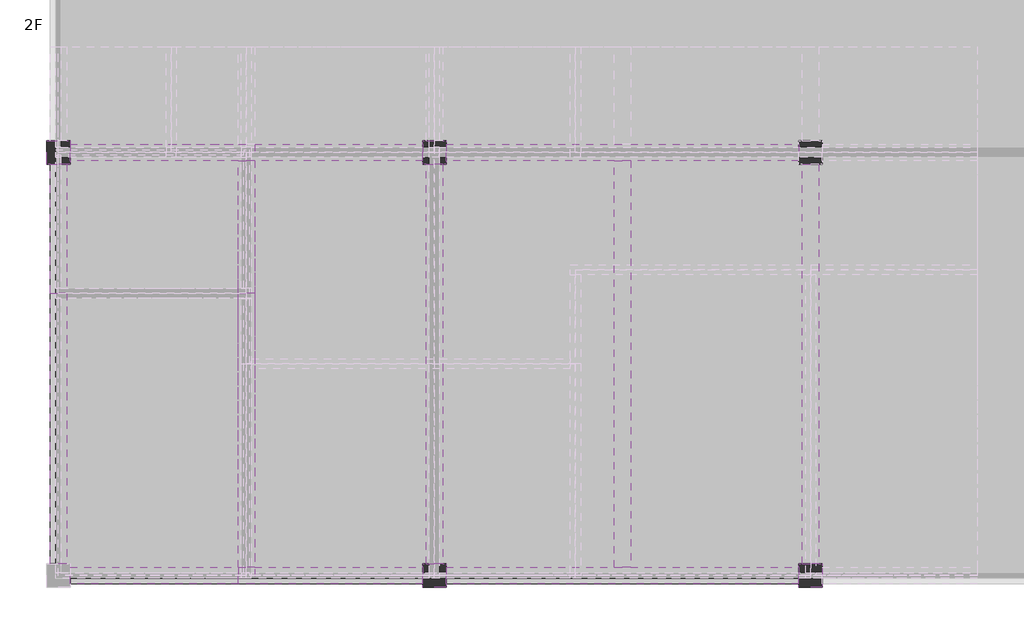
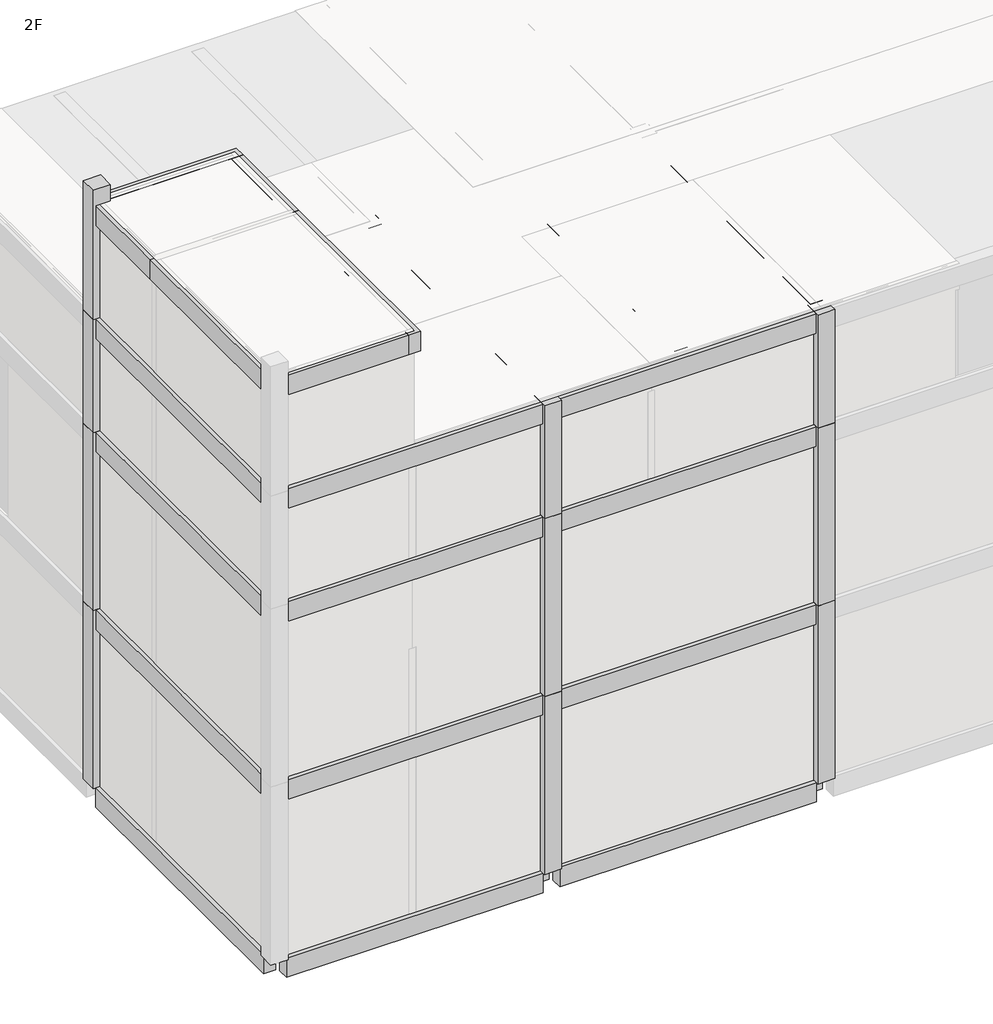
# One storey, part 4 of 7: 42 beams, 14 columns.
"""IFC4 building model written with IfcOpenShell, lengths in millimetres."""

from ifc_helpers import new_model, si_unit, frame, origin, place, context, project, spatial, polyline, outline, extrude, faceted_brep, element, save

model = new_model("IFC4")

# Units and contexts
model_context = context("Model", 3, world=origin())
ifc_project = project(units=[si_unit("LENGTHUNIT", "METRE", prefix="MILLI")], contexts=[model_context])

# Site, building, storey
site = spatial("IfcSite", under=ifc_project)
building = spatial("IfcBuilding", under=site)
storey = spatial("IfcBuildingStorey", under=building, Name="2F", Elevation=3500.0)

# Beams
placement = place(None, origin())
element("IfcBeam", 1, ObjectType="Concrete-Rectangular-Beam : BM111_400x500_RG1", at=placement, inside=storey, context=model_context, shape_type="Brep", body=[
    faceted_brep([(49634.6521483, 169923.8614395, 21500.0), (49284.6521483, 169923.8614395, 21500.0), (49284.6521483, 164098.8614395, 21500.0), (49284.6521483, 163748.8614395, 21500.0), (49634.6521483, 163748.8614395, 21500.0), (49634.6521483, 169923.8614395, 20900.0), (49634.6521483, 163748.8614395, 20900.0), (49284.6521483, 169923.8614395, 20900.0), (49284.6521483, 163748.8614395, 20900.0), (49284.6521483, 164098.8614395, 20900.0)], [[[0, 1, 2, 3, 4]], [[5, 0, 4, 6]], [[7, 5, 6, 8, 9]], [[1, 7, 9, 8, 3, 2]], [[4, 3, 8, 6]], [[1, 0, 5, 7]]]),
])
element("IfcBeam", 2, ObjectType="Concrete-Rectangular-Beam : BM111_400x500_RG1", at=placement, inside=storey, context=model_context, shape_type="SweptSolid", body=[
    extrude(outline(polyline([(49284.6521483, 164098.8614395), (49284.6521483, 163748.8614395), (45709.6521483, 163748.8614395), (45709.6521483, 164098.8614395), (49284.6521483, 164098.8614395)])), frame((0.0, 0.0, 20900.0), z_axis=(0.0, 0.0, 1.0), x_axis=(1.0, 0.0, 0.0)), (0.0, 0.0, 1.0), 600.0),
])
element("IfcBeam", 3, ObjectType="Concrete-Rectangular-Beam : BM111_400x500_RG1", at=placement, inside=storey, context=model_context, shape_type="SweptSolid", body=[
    extrude(outline(polyline([(45284.6521483, 169923.8614395), (45634.6521483, 169923.8614395), (45634.6521483, 164173.8614395), (45284.6521483, 164173.8614395), (45284.6521483, 169923.8614395)])), frame((0.0, 0.0, 20900.0), z_axis=(0.0, 0.0, 1.0), x_axis=(1.0, 0.0, 0.0)), (0.0, 0.0, 1.0), 600.0),
])
element("IfcBeam", 4, ObjectType="Concrete-Rectangular-Beam : BM111_400x500_RG1", at=placement, inside=storey, context=model_context, shape_type="Brep", body=[
    faceted_brep([(49634.6521483, 172748.8614395, 21500.0), (49634.6521483, 173098.8614395, 21500.0), (45709.6521483, 173098.8614395, 21500.0), (45709.6521483, 172748.8614395, 21500.0), (49284.6521483, 172748.8614395, 21500.0), (49634.6521483, 173098.8614395, 20900.0), (45709.6521483, 173098.8614395, 20900.0), (49634.6521483, 172748.8614395, 20900.0), (49284.6521483, 172748.8614395, 20900.0), (45709.6521483, 172748.8614395, 20900.0)], [[[0, 1, 2, 3, 4]], [[1, 5, 6, 2]], [[5, 7, 8, 9, 6]], [[7, 0, 4, 3, 9, 8]], [[3, 2, 6, 9]], [[1, 0, 7, 5]]]),
])
element("IfcBeam", 5, ObjectType="Concrete-Rectangular-Beam : BM111_400x500_RG1", at=placement, inside=storey, context=model_context, shape_type="SweptSolid", body=[
    extrude(outline(polyline([(49634.6521483, 169923.8614395), (49284.6521483, 169923.8614395), (49284.6521483, 172748.8614395), (49634.6521483, 172748.8614395), (49634.6521483, 169923.8614395)])), frame((0.0, 0.0, 20900.0), z_axis=(0.0, 0.0, 1.0), x_axis=(1.0, 0.0, 0.0)), (0.0, 0.0, 1.0), 600.0),
])
element("IfcBeam", 6, ObjectType="Concrete-Rectangular-Beam : BM111_400x500_RG1", at=placement, inside=storey, context=model_context, shape_type="SweptSolid", body=[
    extrude(outline(polyline([(45634.6521483, 169923.8614395), (45284.6521483, 169923.8614395), (45284.6521483, 172673.8614395), (45634.6521483, 172673.8614395), (45634.6521483, 169923.8614395)])), frame((0.0, 0.0, 20900.0), z_axis=(0.0, 0.0, 1.0), x_axis=(1.0, 0.0, 0.0)), (0.0, 0.0, 1.0), 600.0),
])
element("IfcBeam", 7, ObjectType="Concrete-Rectangular-Beam : BM111_400x500_RG1", at=placement, inside=storey, context=model_context, shape_type="SweptSolid", body=[
    extrude(outline(polyline([(49284.6521483, 172748.8614395), (49634.6521483, 172748.8614395), (49634.6521483, 164098.8614395), (49284.6521483, 164098.8614395), (49284.6521483, 172748.8614395)])), frame((0.0, 0.0, 2900.0), z_axis=(0.0, 0.0, 1.0), x_axis=(1.0, 0.0, 0.0)), (0.0, 0.0, 1.0), 600.0),
])
element("IfcBeam", 8, ObjectType="Concrete-Rectangular-Beam : BM111_400x500_RG1", at=placement, inside=storey, context=model_context, shape_type="SweptSolid", body=[
    extrude(outline(polyline([(57284.6521483, 172748.8614395), (57634.6521483, 172748.8614395), (57634.6521483, 164098.8614395), (57284.6521483, 164098.8614395), (57284.6521483, 172748.8614395)])), frame((0.0, 0.0, 2900.0), z_axis=(0.0, 0.0, 1.0), x_axis=(1.0, 0.0, 0.0)), (0.0, 0.0, 1.0), 600.0),
])
element("IfcBeam", 9, ObjectType="Concrete-Rectangular-Beam : BM111_400x500_RG1", at=placement, inside=storey, context=model_context, shape_type="SweptSolid", body=[
    extrude(outline(polyline([(49284.6521483, 172748.8614395), (49634.6521483, 172748.8614395), (49634.6521483, 164098.8614395), (49284.6521483, 164098.8614395), (49284.6521483, 172748.8614395)])), frame((0.0, 0.0, 8400.0), z_axis=(0.0, 0.0, 1.0), x_axis=(1.0, 0.0, 0.0)), (0.0, 0.0, 1.0), 600.0),
])
element("IfcBeam", 10, ObjectType="Concrete-Rectangular-Beam : BM111_400x500_RG1", at=placement, inside=storey, context=model_context, shape_type="SweptSolid", body=[
    extrude(outline(polyline([(57284.6521483, 172748.8614395), (57634.6521483, 172748.8614395), (57634.6521483, 164098.8614395), (57284.6521483, 164098.8614395), (57284.6521483, 172748.8614395)])), frame((0.0, 0.0, 8400.0), z_axis=(0.0, 0.0, 1.0), x_axis=(1.0, 0.0, 0.0)), (0.0, 0.0, 1.0), 600.0),
])
element("IfcBeam", 11, ObjectType="Concrete-Rectangular-Beam : BM111_400x500_RG1", at=placement, inside=storey, context=model_context, shape_type="SweptSolid", body=[
    extrude(outline(polyline([(49284.6521483, 172748.8614395), (49634.6521483, 172748.8614395), (49634.6521483, 164098.8614395), (49284.6521483, 164098.8614395), (49284.6521483, 172748.8614395)])), frame((0.0, 0.0, 13900.0), z_axis=(0.0, 0.0, 1.0), x_axis=(1.0, 0.0, 0.0)), (0.0, 0.0, 1.0), 600.0),
])
element("IfcBeam", 12, ObjectType="Concrete-Rectangular-Beam : BM111_400x500_RG1", at=placement, inside=storey, context=model_context, shape_type="SweptSolid", body=[
    extrude(outline(polyline([(57284.6521483, 172748.8614395), (57634.6521483, 172748.8614395), (57634.6521483, 164098.8614395), (57284.6521483, 164098.8614395), (57284.6521483, 172748.8614395)])), frame((0.0, 0.0, 13900.0), z_axis=(0.0, 0.0, 1.0), x_axis=(1.0, 0.0, 0.0)), (0.0, 0.0, 1.0), 600.0),
])
element("IfcBeam", 13, ObjectType="Concrete-Rectangular-Beam : BM111_400x500_RG1", at=placement, inside=storey, context=model_context, shape_type="SweptSolid", body=[
    extrude(outline(polyline([(49284.6521483, 172748.8614395), (49634.6521483, 172748.8614395), (49634.6521483, 164098.8614395), (49284.6521483, 164098.8614395), (49284.6521483, 172748.8614395)])), frame((0.0, 0.0, 17400.0), z_axis=(0.0, 0.0, 1.0), x_axis=(1.0, 0.0, 0.0)), (0.0, 0.0, 1.0), 600.0),
])
element("IfcBeam", 14, ObjectType="Concrete-Rectangular-Beam : BM111_400x500_RG1", at=placement, inside=storey, context=model_context, shape_type="SweptSolid", body=[
    extrude(outline(polyline([(57284.6521483, 172748.8614395), (57634.6521483, 172748.8614395), (57634.6521483, 164098.8614395), (57284.6521483, 164098.8614395), (57284.6521483, 172748.8614395)])), frame((0.0, 0.0, 17400.0), z_axis=(0.0, 0.0, 1.0), x_axis=(1.0, 0.0, 0.0)), (0.0, 0.0, 1.0), 600.0),
])
element("IfcBeam", 15, ObjectType="Concrete-Rectangular-Beam : BM111_400x500_RG1", at=placement, inside=storey, context=model_context, shape_type="Brep", body=[
    faceted_brep([(45709.6521483, 173098.8614395, 3500.0), (45709.6521483, 172748.8614395, 3500.0), (49284.6521483, 172748.8614395, 3500.0), (49634.6521483, 172748.8614395, 3500.0), (53209.6521483, 172748.8614395, 3500.0), (53209.6521483, 173098.8614395, 3500.0), (49634.6521483, 173098.8614395, 3500.0), (49284.6521483, 173098.8614395, 3500.0), (45709.6521483, 172748.8614395, 2900.0), (49284.6521483, 172748.8614395, 2900.0), (49634.6521483, 172748.8614395, 2900.0), (53209.6521483, 172748.8614395, 2900.0), (45709.6521483, 173098.8614395, 2900.0), (49284.6521483, 173098.8614395, 2900.0), (49634.6521483, 173098.8614395, 2900.0), (53209.6521483, 173098.8614395, 2900.0)], [[[0, 1, 2, 3, 4, 5, 6, 7]], [[1, 8, 9, 10, 11, 4, 3, 2]], [[8, 12, 13, 14, 15, 11, 10, 9]], [[12, 0, 7, 6, 5, 15, 14, 13]], [[1, 0, 12, 8]], [[5, 4, 11, 15]]]),
])
element("IfcBeam", 16, ObjectType="Concrete-Rectangular-Beam : BM111_400x500_RG1", at=placement, inside=storey, context=model_context, shape_type="Brep", body=[
    faceted_brep([(53709.6521483, 173098.8614395, 3500.0), (53709.6521483, 172748.8614395, 3500.0), (57284.6521483, 172748.8614395, 3500.0), (57634.6521483, 172748.8614395, 3500.0), (61209.6521483, 172748.8614395, 3500.0), (61209.6521483, 173098.8614395, 3500.0), (57634.6521483, 173098.8614395, 3500.0), (57284.6521483, 173098.8614395, 3500.0), (53709.6521483, 172748.8614395, 2900.0), (57284.6521483, 172748.8614395, 2900.0), (57634.6521483, 172748.8614395, 2900.0), (61209.6521483, 172748.8614395, 2900.0), (53709.6521483, 173098.8614395, 2900.0), (57284.6521483, 173098.8614395, 2900.0), (57634.6521483, 173098.8614395, 2900.0), (61209.6521483, 173098.8614395, 2900.0)], [[[0, 1, 2, 3, 4, 5, 6, 7]], [[1, 8, 9, 10, 11, 4, 3, 2]], [[8, 12, 13, 14, 15, 11, 10, 9]], [[12, 0, 7, 6, 5, 15, 14, 13]], [[1, 0, 12, 8]], [[5, 4, 11, 15]]]),
])
element("IfcBeam", 17, ObjectType="Concrete-Rectangular-Beam : BM111_400x500_RG1", at=placement, inside=storey, context=model_context, shape_type="Brep", body=[
    faceted_brep([(45709.6521483, 164098.8614395, 3500.0), (45709.6521483, 163748.8614395, 3500.0), (53209.6521483, 163748.8614395, 3500.0), (53209.6521483, 164098.8614395, 3500.0), (49634.6521483, 164098.8614395, 3500.0), (49284.6521483, 164098.8614395, 3500.0), (45709.6521483, 163748.8614395, 2900.0), (53209.6521483, 163748.8614395, 2900.0), (45709.6521483, 164098.8614395, 2900.0), (49284.6521483, 164098.8614395, 2900.0), (49634.6521483, 164098.8614395, 2900.0), (53209.6521483, 164098.8614395, 2900.0)], [[[0, 1, 2, 3, 4, 5]], [[1, 6, 7, 2]], [[6, 8, 9, 10, 11, 7]], [[8, 0, 5, 4, 3, 11, 10, 9]], [[1, 0, 8, 6]], [[3, 2, 7, 11]]]),
])
element("IfcBeam", 18, ObjectType="Concrete-Rectangular-Beam : BM111_400x500_RG1", at=placement, inside=storey, context=model_context, shape_type="Brep", body=[
    faceted_brep([(53709.6521483, 164098.8614395, 3500.0), (53709.6521483, 163748.8614395, 3500.0), (61209.6521483, 163748.8614395, 3500.0), (61209.6521483, 164098.8614395, 3500.0), (57634.6521483, 164098.8614395, 3500.0), (57284.6521483, 164098.8614395, 3500.0), (53709.6521483, 163748.8614395, 2900.0), (61209.6521483, 163748.8614395, 2900.0), (53709.6521483, 164098.8614395, 2900.0), (57284.6521483, 164098.8614395, 2900.0), (57634.6521483, 164098.8614395, 2900.0), (61209.6521483, 164098.8614395, 2900.0)], [[[0, 1, 2, 3, 4, 5]], [[1, 6, 7, 2]], [[6, 8, 9, 10, 11, 7]], [[8, 0, 5, 4, 3, 11, 10, 9]], [[1, 0, 8, 6]], [[3, 2, 7, 11]]]),
])
element("IfcBeam", 19, ObjectType="Concrete-Rectangular-Beam : BM111_400x500_RG1", at=placement, inside=storey, context=model_context, shape_type="Brep", body=[
    faceted_brep([(45709.6521483, 173098.8614395, 9000.0), (45709.6521483, 172748.8614395, 9000.0), (49284.6521483, 172748.8614395, 9000.0), (49634.6521483, 172748.8614395, 9000.0), (53209.6521483, 172748.8614395, 9000.0), (53209.6521483, 173098.8614395, 9000.0), (49634.6521483, 173098.8614395, 9000.0), (49284.6521483, 173098.8614395, 9000.0), (45709.6521483, 172748.8614395, 8400.0), (49284.6521483, 172748.8614395, 8400.0), (49634.6521483, 172748.8614395, 8400.0), (53209.6521483, 172748.8614395, 8400.0), (45709.6521483, 173098.8614395, 8400.0), (49284.6521483, 173098.8614395, 8400.0), (49634.6521483, 173098.8614395, 8400.0), (53209.6521483, 173098.8614395, 8400.0)], [[[0, 1, 2, 3, 4, 5, 6, 7]], [[1, 8, 9, 10, 11, 4, 3, 2]], [[8, 12, 13, 14, 15, 11, 10, 9]], [[12, 0, 7, 6, 5, 15, 14, 13]], [[1, 0, 12, 8]], [[5, 4, 11, 15]]]),
])
element("IfcBeam", 20, ObjectType="Concrete-Rectangular-Beam : BM111_400x500_RG1", at=placement, inside=storey, context=model_context, shape_type="Brep", body=[
    faceted_brep([(53709.6521483, 173098.8614395, 9000.0), (53709.6521483, 172748.8614395, 9000.0), (57284.6521483, 172748.8614395, 9000.0), (57634.6521483, 172748.8614395, 9000.0), (61209.6521483, 172748.8614395, 9000.0), (61209.6521483, 173098.8614395, 9000.0), (57634.6521483, 173098.8614395, 9000.0), (57284.6521483, 173098.8614395, 9000.0), (53709.6521483, 172748.8614395, 8400.0), (57284.6521483, 172748.8614395, 8400.0), (57634.6521483, 172748.8614395, 8400.0), (61209.6521483, 172748.8614395, 8400.0), (53709.6521483, 173098.8614395, 8400.0), (57284.6521483, 173098.8614395, 8400.0), (57634.6521483, 173098.8614395, 8400.0), (61209.6521483, 173098.8614395, 8400.0)], [[[0, 1, 2, 3, 4, 5, 6, 7]], [[1, 8, 9, 10, 11, 4, 3, 2]], [[8, 12, 13, 14, 15, 11, 10, 9]], [[12, 0, 7, 6, 5, 15, 14, 13]], [[1, 0, 12, 8]], [[5, 4, 11, 15]]]),
])
element("IfcBeam", 21, ObjectType="Concrete-Rectangular-Beam : BM111_400x500_RG1", at=placement, inside=storey, context=model_context, shape_type="Brep", body=[
    faceted_brep([(45709.6521483, 164098.8614395, 9000.0), (45709.6521483, 163748.8614395, 9000.0), (53209.6521483, 163748.8614395, 9000.0), (53209.6521483, 164098.8614395, 9000.0), (49634.6521483, 164098.8614395, 9000.0), (49284.6521483, 164098.8614395, 9000.0), (45709.6521483, 163748.8614395, 8400.0), (53209.6521483, 163748.8614395, 8400.0), (45709.6521483, 164098.8614395, 8400.0), (49284.6521483, 164098.8614395, 8400.0), (49634.6521483, 164098.8614395, 8400.0), (53209.6521483, 164098.8614395, 8400.0)], [[[0, 1, 2, 3, 4, 5]], [[1, 6, 7, 2]], [[6, 8, 9, 10, 11, 7]], [[8, 0, 5, 4, 3, 11, 10, 9]], [[1, 0, 8, 6]], [[3, 2, 7, 11]]]),
])
element("IfcBeam", 22, ObjectType="Concrete-Rectangular-Beam : BM111_400x500_RG1", at=placement, inside=storey, context=model_context, shape_type="Brep", body=[
    faceted_brep([(53709.6521483, 164098.8614395, 9000.0), (53709.6521483, 163748.8614395, 9000.0), (61209.6521483, 163748.8614395, 9000.0), (61209.6521483, 164098.8614395, 9000.0), (57634.6521483, 164098.8614395, 9000.0), (57284.6521483, 164098.8614395, 9000.0), (53709.6521483, 163748.8614395, 8400.0), (61209.6521483, 163748.8614395, 8400.0), (53709.6521483, 164098.8614395, 8400.0), (57284.6521483, 164098.8614395, 8400.0), (57634.6521483, 164098.8614395, 8400.0), (61209.6521483, 164098.8614395, 8400.0)], [[[0, 1, 2, 3, 4, 5]], [[1, 6, 7, 2]], [[6, 8, 9, 10, 11, 7]], [[8, 0, 5, 4, 3, 11, 10, 9]], [[1, 0, 8, 6]], [[3, 2, 7, 11]]]),
])
element("IfcBeam", 23, ObjectType="Concrete-Rectangular-Beam : BM111_400x500_RG1", at=placement, inside=storey, context=model_context, shape_type="Brep", body=[
    faceted_brep([(45709.6521483, 173098.8614395, 14500.0), (45709.6521483, 172748.8614395, 14500.0), (49284.6521483, 172748.8614395, 14500.0), (49634.6521483, 172748.8614395, 14500.0), (53209.6521483, 172748.8614395, 14500.0), (53209.6521483, 173098.8614395, 14500.0), (49634.6521483, 173098.8614395, 14500.0), (49284.6521483, 173098.8614395, 14500.0), (45709.6521483, 172748.8614395, 13900.0), (49284.6521483, 172748.8614395, 13900.0), (49634.6521483, 172748.8614395, 13900.0), (53209.6521483, 172748.8614395, 13900.0), (45709.6521483, 173098.8614395, 13900.0), (49284.6521483, 173098.8614395, 13900.0), (49634.6521483, 173098.8614395, 13900.0), (53209.6521483, 173098.8614395, 13900.0)], [[[0, 1, 2, 3, 4, 5, 6, 7]], [[1, 8, 9, 10, 11, 4, 3, 2]], [[8, 12, 13, 14, 15, 11, 10, 9]], [[12, 0, 7, 6, 5, 15, 14, 13]], [[1, 0, 12, 8]], [[5, 4, 11, 15]]]),
])
element("IfcBeam", 24, ObjectType="Concrete-Rectangular-Beam : BM111_400x500_RG1", at=placement, inside=storey, context=model_context, shape_type="Brep", body=[
    faceted_brep([(53709.6521483, 173098.8614395, 14500.0), (53709.6521483, 172748.8614395, 14500.0), (57284.6521483, 172748.8614395, 14500.0), (57634.6521483, 172748.8614395, 14500.0), (61209.6521483, 172748.8614395, 14500.0), (61209.6521483, 173098.8614395, 14500.0), (57634.6521483, 173098.8614395, 14500.0), (57284.6521483, 173098.8614395, 14500.0), (53709.6521483, 172748.8614395, 13900.0), (57284.6521483, 172748.8614395, 13900.0), (57634.6521483, 172748.8614395, 13900.0), (61209.6521483, 172748.8614395, 13900.0), (53709.6521483, 173098.8614395, 13900.0), (57284.6521483, 173098.8614395, 13900.0), (57634.6521483, 173098.8614395, 13900.0), (61209.6521483, 173098.8614395, 13900.0)], [[[0, 1, 2, 3, 4, 5, 6, 7]], [[1, 8, 9, 10, 11, 4, 3, 2]], [[8, 12, 13, 14, 15, 11, 10, 9]], [[12, 0, 7, 6, 5, 15, 14, 13]], [[1, 0, 12, 8]], [[5, 4, 11, 15]]]),
])
element("IfcBeam", 25, ObjectType="Concrete-Rectangular-Beam : BM111_400x500_RG1", at=placement, inside=storey, context=model_context, shape_type="Brep", body=[
    faceted_brep([(45709.6521483, 164098.8614395, 14500.0), (45709.6521483, 163748.8614395, 14500.0), (53209.6521483, 163748.8614395, 14500.0), (53209.6521483, 164098.8614395, 14500.0), (49634.6521483, 164098.8614395, 14500.0), (49284.6521483, 164098.8614395, 14500.0), (45709.6521483, 163748.8614395, 13900.0), (53209.6521483, 163748.8614395, 13900.0), (45709.6521483, 164098.8614395, 13900.0), (49284.6521483, 164098.8614395, 13900.0), (49634.6521483, 164098.8614395, 13900.0), (53209.6521483, 164098.8614395, 13900.0)], [[[0, 1, 2, 3, 4, 5]], [[1, 6, 7, 2]], [[6, 8, 9, 10, 11, 7]], [[8, 0, 5, 4, 3, 11, 10, 9]], [[1, 0, 8, 6]], [[3, 2, 7, 11]]]),
])
element("IfcBeam", 26, ObjectType="Concrete-Rectangular-Beam : BM111_400x500_RG1", at=placement, inside=storey, context=model_context, shape_type="Brep", body=[
    faceted_brep([(53709.6521483, 164098.8614395, 14500.0), (53709.6521483, 163748.8614395, 14500.0), (61209.6521483, 163748.8614395, 14500.0), (61209.6521483, 164098.8614395, 14500.0), (57634.6521483, 164098.8614395, 14500.0), (57284.6521483, 164098.8614395, 14500.0), (53709.6521483, 163748.8614395, 13900.0), (61209.6521483, 163748.8614395, 13900.0), (53709.6521483, 164098.8614395, 13900.0), (57284.6521483, 164098.8614395, 13900.0), (57634.6521483, 164098.8614395, 13900.0), (61209.6521483, 164098.8614395, 13900.0)], [[[0, 1, 2, 3, 4, 5]], [[1, 6, 7, 2]], [[6, 8, 9, 10, 11, 7]], [[8, 0, 5, 4, 3, 11, 10, 9]], [[1, 0, 8, 6]], [[3, 2, 7, 11]]]),
])
element("IfcBeam", 27, ObjectType="Concrete-Rectangular-Beam : BM111_400x500_RG1", at=placement, inside=storey, context=model_context, shape_type="Brep", body=[
    faceted_brep([(45709.6521483, 173098.8614395, 18000.0), (45709.6521483, 172748.8614395, 18000.0), (49284.6521483, 172748.8614395, 18000.0), (49634.6521483, 172748.8614395, 18000.0), (53209.6521483, 172748.8614395, 18000.0), (53209.6521483, 173098.8614395, 18000.0), (49634.6521483, 173098.8614395, 18000.0), (49284.6521483, 173098.8614395, 18000.0), (45709.6521483, 172748.8614395, 17400.0), (49284.6521483, 172748.8614395, 17400.0), (49634.6521483, 172748.8614395, 17400.0), (53209.6521483, 172748.8614395, 17400.0), (45709.6521483, 173098.8614395, 17400.0), (49284.6521483, 173098.8614395, 17400.0), (49634.6521483, 173098.8614395, 17400.0), (53209.6521483, 173098.8614395, 17400.0)], [[[0, 1, 2, 3, 4, 5, 6, 7]], [[1, 8, 9, 10, 11, 4, 3, 2]], [[8, 12, 13, 14, 15, 11, 10, 9]], [[12, 0, 7, 6, 5, 15, 14, 13]], [[1, 0, 12, 8]], [[5, 4, 11, 15]]]),
])
element("IfcBeam", 28, ObjectType="Concrete-Rectangular-Beam : BM111_400x500_RG1", at=placement, inside=storey, context=model_context, shape_type="Brep", body=[
    faceted_brep([(53709.6521483, 173098.8614395, 18000.0), (53709.6521483, 172748.8614395, 18000.0), (57284.6521483, 172748.8614395, 18000.0), (57634.6521483, 172748.8614395, 18000.0), (61209.6521483, 172748.8614395, 18000.0), (61209.6521483, 173098.8614395, 18000.0), (57634.6521483, 173098.8614395, 18000.0), (57284.6521483, 173098.8614395, 18000.0), (53709.6521483, 172748.8614395, 17400.0), (57284.6521483, 172748.8614395, 17400.0), (57634.6521483, 172748.8614395, 17400.0), (61209.6521483, 172748.8614395, 17400.0), (53709.6521483, 173098.8614395, 17400.0), (57284.6521483, 173098.8614395, 17400.0), (57634.6521483, 173098.8614395, 17400.0), (61209.6521483, 173098.8614395, 17400.0)], [[[0, 1, 2, 3, 4, 5, 6, 7]], [[1, 8, 9, 10, 11, 4, 3, 2]], [[8, 12, 13, 14, 15, 11, 10, 9]], [[12, 0, 7, 6, 5, 15, 14, 13]], [[1, 0, 12, 8]], [[5, 4, 11, 15]]]),
])
element("IfcBeam", 29, ObjectType="Concrete-Rectangular-Beam : BM111_400x500_RG1", at=placement, inside=storey, context=model_context, shape_type="Brep", body=[
    faceted_brep([(45709.6521483, 164098.8614395, 18000.0), (45709.6521483, 163748.8614395, 18000.0), (53209.6521483, 163748.8614395, 18000.0), (53209.6521483, 164098.8614395, 18000.0), (49634.6521483, 164098.8614395, 18000.0), (49284.6521483, 164098.8614395, 18000.0), (45709.6521483, 163748.8614395, 17400.0), (53209.6521483, 163748.8614395, 17400.0), (45709.6521483, 164098.8614395, 17400.0), (49284.6521483, 164098.8614395, 17400.0), (49634.6521483, 164098.8614395, 17400.0), (53209.6521483, 164098.8614395, 17400.0)], [[[0, 1, 2, 3, 4, 5]], [[1, 6, 7, 2]], [[6, 8, 9, 10, 11, 7]], [[8, 0, 5, 4, 3, 11, 10, 9]], [[1, 0, 8, 6]], [[3, 2, 7, 11]]]),
])
element("IfcBeam", 30, ObjectType="Concrete-Rectangular-Beam : BM111_400x500_RG1", at=placement, inside=storey, context=model_context, shape_type="Brep", body=[
    faceted_brep([(53709.6521483, 164098.8614395, 18000.0), (53709.6521483, 163748.8614395, 18000.0), (61209.6521483, 163748.8614395, 18000.0), (61209.6521483, 164098.8614395, 18000.0), (57634.6521483, 164098.8614395, 18000.0), (57284.6521483, 164098.8614395, 18000.0), (53709.6521483, 163748.8614395, 17400.0), (61209.6521483, 163748.8614395, 17400.0), (53709.6521483, 164098.8614395, 17400.0), (57284.6521483, 164098.8614395, 17400.0), (57634.6521483, 164098.8614395, 17400.0), (61209.6521483, 164098.8614395, 17400.0)], [[[0, 1, 2, 3, 4, 5]], [[1, 6, 7, 2]], [[6, 8, 9, 10, 11, 7]], [[8, 0, 5, 4, 3, 11, 10, 9]], [[1, 0, 8, 6]], [[3, 2, 7, 11]]]),
])
element("IfcBeam", 31, ObjectType="Concrete-Rectangular-Beam : BM111_400x500_RG1", at=placement, inside=storey, context=model_context, shape_type="SweptSolid", body=[
    extrude(outline(polyline([(45284.6521483, 172673.8614395), (45634.6521483, 172673.8614395), (45634.6521483, 164173.8614395), (45284.6521483, 164173.8614395), (45284.6521483, 172673.8614395)])), frame((0.0, 0.0, 2900.0), z_axis=(0.0, 0.0, 1.0), x_axis=(1.0, 0.0, 0.0)), (0.0, 0.0, 1.0), 600.0),
])
element("IfcBeam", 32, ObjectType="Concrete-Rectangular-Beam : BM111_400x500_RG1", at=placement, inside=storey, context=model_context, shape_type="SweptSolid", body=[
    extrude(outline(polyline([(53284.6521483, 172673.8614395), (53634.6521483, 172673.8614395), (53634.6521483, 164173.8614395), (53284.6521483, 164173.8614395), (53284.6521483, 172673.8614395)])), frame((0.0, 0.0, 2900.0), z_axis=(0.0, 0.0, 1.0), x_axis=(1.0, 0.0, 0.0)), (0.0, 0.0, 1.0), 600.0),
])
element("IfcBeam", 33, ObjectType="Concrete-Rectangular-Beam : BM111_400x500_RG1", at=placement, inside=storey, context=model_context, shape_type="SweptSolid", body=[
    extrude(outline(polyline([(61284.6521483, 172673.8614395), (61634.6521483, 172673.8614395), (61634.6521483, 164173.8614395), (61284.6521483, 164173.8614395), (61284.6521483, 172673.8614395)])), frame((0.0, 0.0, 2900.0), z_axis=(0.0, 0.0, 1.0), x_axis=(1.0, 0.0, 0.0)), (0.0, 0.0, 1.0), 600.0),
])
element("IfcBeam", 34, ObjectType="Concrete-Rectangular-Beam : BM111_400x500_RG1", at=placement, inside=storey, context=model_context, shape_type="SweptSolid", body=[
    extrude(outline(polyline([(45284.6521483, 172673.8614395), (45634.6521483, 172673.8614395), (45634.6521483, 164173.8614395), (45284.6521483, 164173.8614395), (45284.6521483, 172673.8614395)])), frame((0.0, 0.0, 8400.0), z_axis=(0.0, 0.0, 1.0), x_axis=(1.0, 0.0, 0.0)), (0.0, 0.0, 1.0), 600.0),
])
element("IfcBeam", 35, ObjectType="Concrete-Rectangular-Beam : BM111_400x500_RG1", at=placement, inside=storey, context=model_context, shape_type="SweptSolid", body=[
    extrude(outline(polyline([(53284.6521483, 172673.8614395), (53634.6521483, 172673.8614395), (53634.6521483, 164173.8614395), (53284.6521483, 164173.8614395), (53284.6521483, 172673.8614395)])), frame((0.0, 0.0, 8400.0), z_axis=(0.0, 0.0, 1.0), x_axis=(1.0, 0.0, 0.0)), (0.0, 0.0, 1.0), 600.0),
])
element("IfcBeam", 36, ObjectType="Concrete-Rectangular-Beam : BM111_400x500_RG1", at=placement, inside=storey, context=model_context, shape_type="SweptSolid", body=[
    extrude(outline(polyline([(61284.6521483, 172673.8614395), (61634.6521483, 172673.8614395), (61634.6521483, 164173.8614395), (61284.6521483, 164173.8614395), (61284.6521483, 172673.8614395)])), frame((0.0, 0.0, 8400.0), z_axis=(0.0, 0.0, 1.0), x_axis=(1.0, 0.0, 0.0)), (0.0, 0.0, 1.0), 600.0),
])
element("IfcBeam", 37, ObjectType="Concrete-Rectangular-Beam : BM111_400x500_RG1", at=placement, inside=storey, context=model_context, shape_type="SweptSolid", body=[
    extrude(outline(polyline([(45284.6521483, 172673.8614395), (45634.6521483, 172673.8614395), (45634.6521483, 164173.8614395), (45284.6521483, 164173.8614395), (45284.6521483, 172673.8614395)])), frame((0.0, 0.0, 13900.0), z_axis=(0.0, 0.0, 1.0), x_axis=(1.0, 0.0, 0.0)), (0.0, 0.0, 1.0), 600.0),
])
element("IfcBeam", 38, ObjectType="Concrete-Rectangular-Beam : BM111_400x500_RG1", at=placement, inside=storey, context=model_context, shape_type="SweptSolid", body=[
    extrude(outline(polyline([(53284.6521483, 172673.8614395), (53634.6521483, 172673.8614395), (53634.6521483, 164173.8614395), (53284.6521483, 164173.8614395), (53284.6521483, 172673.8614395)])), frame((0.0, 0.0, 13900.0), z_axis=(0.0, 0.0, 1.0), x_axis=(1.0, 0.0, 0.0)), (0.0, 0.0, 1.0), 600.0),
])
element("IfcBeam", 39, ObjectType="Concrete-Rectangular-Beam : BM111_400x500_RG1", at=placement, inside=storey, context=model_context, shape_type="SweptSolid", body=[
    extrude(outline(polyline([(61284.6521483, 172673.8614395), (61634.6521483, 172673.8614395), (61634.6521483, 164173.8614395), (61284.6521483, 164173.8614395), (61284.6521483, 172673.8614395)])), frame((0.0, 0.0, 13900.0), z_axis=(0.0, 0.0, 1.0), x_axis=(1.0, 0.0, 0.0)), (0.0, 0.0, 1.0), 600.0),
])
element("IfcBeam", 40, ObjectType="Concrete-Rectangular-Beam : BM111_400x500_RG1", at=placement, inside=storey, context=model_context, shape_type="SweptSolid", body=[
    extrude(outline(polyline([(45284.6521483, 172673.8614395), (45634.6521483, 172673.8614395), (45634.6521483, 164173.8614395), (45284.6521483, 164173.8614395), (45284.6521483, 172673.8614395)])), frame((0.0, 0.0, 17400.0), z_axis=(0.0, 0.0, 1.0), x_axis=(1.0, 0.0, 0.0)), (0.0, 0.0, 1.0), 600.0),
])
element("IfcBeam", 41, ObjectType="Concrete-Rectangular-Beam : BM111_400x500_RG1", at=placement, inside=storey, context=model_context, shape_type="SweptSolid", body=[
    extrude(outline(polyline([(53284.6521483, 172673.8614395), (53634.6521483, 172673.8614395), (53634.6521483, 164173.8614395), (53284.6521483, 164173.8614395), (53284.6521483, 172673.8614395)])), frame((0.0, 0.0, 17400.0), z_axis=(0.0, 0.0, 1.0), x_axis=(1.0, 0.0, 0.0)), (0.0, 0.0, 1.0), 600.0),
])
element("IfcBeam", 42, ObjectType="Concrete-Rectangular-Beam : BM111_400x500_RG1", at=placement, inside=storey, context=model_context, shape_type="SweptSolid", body=[
    extrude(outline(polyline([(61284.6521483, 172673.8614395), (61634.6521483, 172673.8614395), (61634.6521483, 164173.8614395), (61284.6521483, 164173.8614395), (61284.6521483, 172673.8614395)])), frame((0.0, 0.0, 17400.0), z_axis=(0.0, 0.0, 1.0), x_axis=(1.0, 0.0, 0.0)), (0.0, 0.0, 1.0), 600.0),
])

# Columns
element("IfcColumn", 43, ObjectType="Concrete-Rectangular-Column : CL111_500x500", at=placement, inside=storey, context=model_context, shape_type="SweptSolid", body=[
    extrude(outline(polyline([(45709.6521483, 173173.8614395), (45709.6521483, 172673.8614395), (45209.6521483, 172673.8614395), (45209.6521483, 173173.8614395), (45709.6521483, 173173.8614395)])), frame((0.0, 0.0, 18000.0), z_axis=(0.0, 0.0, 1.0), x_axis=(1.0, 0.0, 0.0)), (0.0, 0.0, 1.0), 4000.0),
])
element("IfcColumn", 44, ObjectType="Concrete-Rectangular-Column : CL111_500x500", at=placement, inside=storey, context=model_context, shape_type="Brep", body=[
    faceted_brep([(45709.6521483, 173173.8614395, 3500.0), (45709.6521483, 172673.8614395, 3500.0), (45209.6521483, 172673.8614395, 3500.0), (45209.6521483, 173173.8614395, 3500.0), (45709.6521483, 173173.8614395, 9000.0), (45709.6521483, 173098.8614395, 9000.0), (45709.6521483, 172748.8614395, 9000.0), (45709.6521483, 172673.8614395, 9000.0), (45634.6521483, 172673.8614395, 9000.0), (45284.6521483, 172673.8614395, 9000.0), (45209.6521483, 172673.8614395, 9000.0), (45209.6521483, 173173.8614395, 9000.0), (45284.6521483, 173173.8614395, 9000.0), (45634.6521483, 173173.8614395, 9000.0)], [[[0, 1, 2, 3]], [[4, 5, 6, 7, 1, 0]], [[7, 8, 9, 10, 2, 1]], [[10, 11, 3, 2]], [[11, 12, 13, 4, 0, 3]], [[4, 13, 12, 11, 10, 9, 8, 7, 6, 5]]]),
])
element("IfcColumn", 45, ObjectType="Concrete-Rectangular-Column : CL111_500x500", at=placement, inside=storey, context=model_context, shape_type="Brep", body=[
    faceted_brep([(45709.6521483, 173173.8614395, 9000.0), (45709.6521483, 172673.8614395, 9000.0), (45209.6521483, 172673.8614395, 9000.0), (45209.6521483, 173173.8614395, 9000.0), (45709.6521483, 173173.8614395, 14500.0), (45709.6521483, 173098.8614395, 14500.0), (45709.6521483, 172748.8614395, 14500.0), (45709.6521483, 172673.8614395, 14500.0), (45634.6521483, 172673.8614395, 14500.0), (45284.6521483, 172673.8614395, 14500.0), (45209.6521483, 172673.8614395, 14500.0), (45209.6521483, 173173.8614395, 14500.0), (45284.6521483, 173173.8614395, 14500.0), (45634.6521483, 173173.8614395, 14500.0)], [[[0, 1, 2, 3]], [[4, 5, 6, 7, 1, 0]], [[7, 8, 9, 10, 2, 1]], [[10, 11, 3, 2]], [[11, 12, 13, 4, 0, 3]], [[4, 13, 12, 11, 10, 9, 8, 7, 6, 5]]]),
])
element("IfcColumn", 46, ObjectType="Concrete-Rectangular-Column : CL111_500x500", at=placement, inside=storey, context=model_context, shape_type="Brep", body=[
    faceted_brep([(45709.6521483, 173173.8614395, 14500.0), (45709.6521483, 172673.8614395, 14500.0), (45209.6521483, 172673.8614395, 14500.0), (45209.6521483, 173173.8614395, 14500.0), (45709.6521483, 173173.8614395, 18000.0), (45709.6521483, 173098.8614395, 18000.0), (45709.6521483, 172748.8614395, 18000.0), (45709.6521483, 172673.8614395, 18000.0), (45634.6521483, 172673.8614395, 18000.0), (45284.6521483, 172673.8614395, 18000.0), (45209.6521483, 172673.8614395, 18000.0), (45209.6521483, 173173.8614395, 18000.0), (45284.6521483, 173173.8614395, 18000.0), (45634.6521483, 173173.8614395, 18000.0)], [[[0, 1, 2, 3]], [[4, 5, 6, 7, 1, 0]], [[7, 8, 9, 10, 2, 1]], [[10, 11, 3, 2]], [[11, 12, 13, 4, 0, 3]], [[4, 13, 12, 11, 10, 9, 8, 7, 6, 5]]]),
])
element("IfcColumn", 47, ObjectType="Concrete-Rectangular-Column : CL111_500x500", at=placement, inside=storey, context=model_context, shape_type="Brep", body=[
    faceted_brep([(53709.6521483, 173173.8614395, 3500.0), (53709.6521483, 172673.8614395, 3500.0), (53209.6521483, 172673.8614395, 3500.0), (53209.6521483, 173173.8614395, 3500.0), (53709.6521483, 173173.8614395, 9000.0), (53709.6521483, 173098.8614395, 9000.0), (53709.6521483, 172748.8614395, 9000.0), (53709.6521483, 172673.8614395, 9000.0), (53634.6521483, 172673.8614395, 9000.0), (53284.6521483, 172673.8614395, 9000.0), (53209.6521483, 172673.8614395, 9000.0), (53209.6521483, 172748.8614395, 9000.0), (53209.6521483, 173098.8614395, 9000.0), (53209.6521483, 173173.8614395, 9000.0), (53284.6521483, 173173.8614395, 9000.0), (53634.6521483, 173173.8614395, 9000.0)], [[[0, 1, 2, 3]], [[4, 5, 6, 7, 1, 0]], [[7, 8, 9, 10, 2, 1]], [[10, 11, 12, 13, 3, 2]], [[13, 14, 15, 4, 0, 3]], [[4, 15, 14, 13, 12, 11, 10, 9, 8, 7, 6, 5]]]),
])
element("IfcColumn", 48, ObjectType="Concrete-Rectangular-Column : CL111_500x500", at=placement, inside=storey, context=model_context, shape_type="Brep", body=[
    faceted_brep([(53709.6521483, 173173.8614395, 9000.0), (53709.6521483, 172673.8614395, 9000.0), (53209.6521483, 172673.8614395, 9000.0), (53209.6521483, 173173.8614395, 9000.0), (53709.6521483, 173173.8614395, 14500.0), (53709.6521483, 173098.8614395, 14500.0), (53709.6521483, 172748.8614395, 14500.0), (53709.6521483, 172673.8614395, 14500.0), (53634.6521483, 172673.8614395, 14500.0), (53284.6521483, 172673.8614395, 14500.0), (53209.6521483, 172673.8614395, 14500.0), (53209.6521483, 172748.8614395, 14500.0), (53209.6521483, 173098.8614395, 14500.0), (53209.6521483, 173173.8614395, 14500.0), (53284.6521483, 173173.8614395, 14500.0), (53634.6521483, 173173.8614395, 14500.0)], [[[0, 1, 2, 3]], [[4, 5, 6, 7, 1, 0]], [[7, 8, 9, 10, 2, 1]], [[10, 11, 12, 13, 3, 2]], [[13, 14, 15, 4, 0, 3]], [[4, 15, 14, 13, 12, 11, 10, 9, 8, 7, 6, 5]]]),
])
element("IfcColumn", 49, ObjectType="Concrete-Rectangular-Column : CL111_500x500", at=placement, inside=storey, context=model_context, shape_type="Brep", body=[
    faceted_brep([(53709.6521483, 173173.8614395, 14500.0), (53709.6521483, 172673.8614395, 14500.0), (53209.6521483, 172673.8614395, 14500.0), (53209.6521483, 173173.8614395, 14500.0), (53709.6521483, 173173.8614395, 18000.0), (53709.6521483, 173098.8614395, 18000.0), (53709.6521483, 172748.8614395, 18000.0), (53709.6521483, 172673.8614395, 18000.0), (53634.6521483, 172673.8614395, 18000.0), (53284.6521483, 172673.8614395, 18000.0), (53209.6521483, 172673.8614395, 18000.0), (53209.6521483, 172748.8614395, 18000.0), (53209.6521483, 173098.8614395, 18000.0), (53209.6521483, 173173.8614395, 18000.0), (53284.6521483, 173173.8614395, 18000.0), (53634.6521483, 173173.8614395, 18000.0)], [[[0, 1, 2, 3]], [[4, 5, 6, 7, 1, 0]], [[7, 8, 9, 10, 2, 1]], [[10, 11, 12, 13, 3, 2]], [[13, 14, 15, 4, 0, 3]], [[4, 15, 14, 13, 12, 11, 10, 9, 8, 7, 6, 5]]]),
])
element("IfcColumn", 50, ObjectType="Concrete-Rectangular-Column : CL111_500x500", at=placement, inside=storey, context=model_context, shape_type="Brep", body=[
    faceted_brep([(61709.6521483, 173173.8614395, 3500.0), (61709.6521483, 172673.8614395, 3500.0), (61209.6521483, 172673.8614395, 3500.0), (61209.6521483, 173173.8614395, 3500.0), (61709.6521483, 173173.8614395, 9000.0), (61709.6521483, 173098.8614395, 9000.0), (61709.6521483, 172748.8614395, 9000.0), (61709.6521483, 172673.8614395, 9000.0), (61634.6521483, 172673.8614395, 9000.0), (61284.6521483, 172673.8614395, 9000.0), (61209.6521483, 172673.8614395, 9000.0), (61209.6521483, 172748.8614395, 9000.0), (61209.6521483, 173098.8614395, 9000.0), (61209.6521483, 173173.8614395, 9000.0), (61284.6521483, 173173.8614395, 9000.0), (61634.6521483, 173173.8614395, 9000.0)], [[[0, 1, 2, 3]], [[4, 5, 6, 7, 1, 0]], [[7, 8, 9, 10, 2, 1]], [[10, 11, 12, 13, 3, 2]], [[13, 14, 15, 4, 0, 3]], [[4, 15, 14, 13, 12, 11, 10, 9, 8, 7, 6, 5]]]),
])
element("IfcColumn", 51, ObjectType="Concrete-Rectangular-Column : CL111_500x500", at=placement, inside=storey, context=model_context, shape_type="Brep", body=[
    faceted_brep([(53709.6521483, 164173.8614395, 3500.0), (53709.6521483, 163673.8614395, 3500.0), (53209.6521483, 163673.8614395, 3500.0), (53209.6521483, 164173.8614395, 3500.0), (53709.6521483, 164173.8614395, 9000.0), (53709.6521483, 164098.8614395, 9000.0), (53709.6521483, 163748.8614395, 9000.0), (53709.6521483, 163673.8614395, 9000.0), (53209.6521483, 163673.8614395, 9000.0), (53209.6521483, 163748.8614395, 9000.0), (53209.6521483, 164098.8614395, 9000.0), (53209.6521483, 164173.8614395, 9000.0), (53284.6521483, 164173.8614395, 9000.0), (53634.6521483, 164173.8614395, 9000.0)], [[[0, 1, 2, 3]], [[4, 5, 6, 7, 1, 0]], [[7, 8, 2, 1]], [[8, 9, 10, 11, 3, 2]], [[11, 12, 13, 4, 0, 3]], [[4, 13, 12, 11, 10, 9, 8, 7, 6, 5]]]),
])
element("IfcColumn", 52, ObjectType="Concrete-Rectangular-Column : CL111_500x500", at=placement, inside=storey, context=model_context, shape_type="Brep", body=[
    faceted_brep([(53709.6521483, 164173.8614395, 9000.0), (53709.6521483, 163673.8614395, 9000.0), (53209.6521483, 163673.8614395, 9000.0), (53209.6521483, 164173.8614395, 9000.0), (53709.6521483, 164173.8614395, 14500.0), (53709.6521483, 164098.8614395, 14500.0), (53709.6521483, 163748.8614395, 14500.0), (53709.6521483, 163673.8614395, 14500.0), (53209.6521483, 163673.8614395, 14500.0), (53209.6521483, 163748.8614395, 14500.0), (53209.6521483, 164098.8614395, 14500.0), (53209.6521483, 164173.8614395, 14500.0), (53284.6521483, 164173.8614395, 14500.0), (53634.6521483, 164173.8614395, 14500.0)], [[[0, 1, 2, 3]], [[4, 5, 6, 7, 1, 0]], [[7, 8, 2, 1]], [[8, 9, 10, 11, 3, 2]], [[11, 12, 13, 4, 0, 3]], [[4, 13, 12, 11, 10, 9, 8, 7, 6, 5]]]),
])
element("IfcColumn", 53, ObjectType="Concrete-Rectangular-Column : CL111_500x500", at=placement, inside=storey, context=model_context, shape_type="Brep", body=[
    faceted_brep([(53709.6521483, 164173.8614395, 14500.0), (53709.6521483, 163673.8614395, 14500.0), (53209.6521483, 163673.8614395, 14500.0), (53209.6521483, 164173.8614395, 14500.0), (53709.6521483, 164173.8614395, 18000.0), (53709.6521483, 164098.8614395, 18000.0), (53709.6521483, 163748.8614395, 18000.0), (53709.6521483, 163673.8614395, 18000.0), (53209.6521483, 163673.8614395, 18000.0), (53209.6521483, 163748.8614395, 18000.0), (53209.6521483, 164098.8614395, 18000.0), (53209.6521483, 164173.8614395, 18000.0), (53284.6521483, 164173.8614395, 18000.0), (53634.6521483, 164173.8614395, 18000.0)], [[[0, 1, 2, 3]], [[4, 5, 6, 7, 1, 0]], [[7, 8, 2, 1]], [[8, 9, 10, 11, 3, 2]], [[11, 12, 13, 4, 0, 3]], [[4, 13, 12, 11, 10, 9, 8, 7, 6, 5]]]),
])
element("IfcColumn", 54, ObjectType="Concrete-Rectangular-Column : CL111_500x500", at=placement, inside=storey, context=model_context, shape_type="Brep", body=[
    faceted_brep([(61709.6521483, 164173.8614395, 3500.0), (61709.6521483, 163673.8614395, 3500.0), (61209.6521483, 163673.8614395, 3500.0), (61209.6521483, 164173.8614395, 3500.0), (61709.6521483, 164173.8614395, 9000.0), (61709.6521483, 164098.8614395, 9000.0), (61709.6521483, 163748.8614395, 9000.0), (61709.6521483, 163673.8614395, 9000.0), (61209.6521483, 163673.8614395, 9000.0), (61209.6521483, 163748.8614395, 9000.0), (61209.6521483, 164098.8614395, 9000.0), (61209.6521483, 164173.8614395, 9000.0), (61284.6521483, 164173.8614395, 9000.0), (61634.6521483, 164173.8614395, 9000.0)], [[[0, 1, 2, 3]], [[4, 5, 6, 7, 1, 0]], [[7, 8, 2, 1]], [[8, 9, 10, 11, 3, 2]], [[11, 12, 13, 4, 0, 3]], [[4, 13, 12, 11, 10, 9, 8, 7, 6, 5]]]),
])
element("IfcColumn", 55, ObjectType="Concrete-Rectangular-Column : CL111_500x500", at=placement, inside=storey, context=model_context, shape_type="Brep", body=[
    faceted_brep([(61709.6521483, 164173.8614395, 9000.0), (61709.6521483, 163673.8614395, 9000.0), (61209.6521483, 163673.8614395, 9000.0), (61209.6521483, 164173.8614395, 9000.0), (61709.6521483, 164173.8614395, 14500.0), (61709.6521483, 164098.8614395, 14500.0), (61709.6521483, 163748.8614395, 14500.0), (61709.6521483, 163673.8614395, 14500.0), (61209.6521483, 163673.8614395, 14500.0), (61209.6521483, 163748.8614395, 14500.0), (61209.6521483, 164098.8614395, 14500.0), (61209.6521483, 164173.8614395, 14500.0), (61284.6521483, 164173.8614395, 14500.0), (61634.6521483, 164173.8614395, 14500.0)], [[[0, 1, 2, 3]], [[4, 5, 6, 7, 1, 0]], [[7, 8, 2, 1]], [[8, 9, 10, 11, 3, 2]], [[11, 12, 13, 4, 0, 3]], [[4, 13, 12, 11, 10, 9, 8, 7, 6, 5]]]),
])
element("IfcColumn", 56, ObjectType="Concrete-Rectangular-Column : CL111_500x500", at=placement, inside=storey, context=model_context, shape_type="Brep", body=[
    faceted_brep([(61709.6521483, 164173.8614395, 14500.0), (61709.6521483, 163673.8614395, 14500.0), (61209.6521483, 163673.8614395, 14500.0), (61209.6521483, 164173.8614395, 14500.0), (61709.6521483, 164173.8614395, 18000.0), (61709.6521483, 164098.8614395, 18000.0), (61709.6521483, 163748.8614395, 18000.0), (61709.6521483, 163673.8614395, 18000.0), (61209.6521483, 163673.8614395, 18000.0), (61209.6521483, 163748.8614395, 18000.0), (61209.6521483, 164098.8614395, 18000.0), (61209.6521483, 164173.8614395, 18000.0), (61284.6521483, 164173.8614395, 18000.0), (61634.6521483, 164173.8614395, 18000.0)], [[[0, 1, 2, 3]], [[4, 5, 6, 7, 1, 0]], [[7, 8, 2, 1]], [[8, 9, 10, 11, 3, 2]], [[11, 12, 13, 4, 0, 3]], [[4, 13, 12, 11, 10, 9, 8, 7, 6, 5]]]),
])

save(model, "model.ifc")

# Revit data of these elements
# Type "Concrete-Rectangular-Beam : BM111_400x500_RG1"
#   중앙부 하부근 = "3-D20"
#   중앙부 상부근 = "3-D20"
#   중앙부 보조근 = ""
#   중앙부 늑근 = "2-D10 @200"
#   외단부 하부근 = "3-D20"
#   외단부 상부근 = "3-D20"
#   외단부 보조근 = ""
#   외단부 늑근 = "2-D10 @100"
#   부호 = "RG1"
#   내단부 하부근 = "3-D20"
#   내단부 상부근 = "3-D20"
#   내단부 보조근 = ""
#   내단부 늑근 = "2-D10 @100"
#   ALL 하부근 = ""
#   ALL 상부근 = ""
#   ALL 보조근 = ""
#   ALL 늑근 = ""
#   Width = 400 mm
#   Height = 500 mm
#   Length [instance default] = 1524 mm
#   Structural Material [instance default] = 콘크리트 - 현장타설 콘크리트
#   hec_material3 [instance default] = none
#   hec_material2 [instance default] = none
#   hec_material1 [instance default] = none
#   Assembly Code = ""
# Type "Concrete-Rectangular-Column : CL111_500x500"
#   Description = "UG 철골 기둥용 Pedestal"
#   b = 500 mm
#   h = 500 mm
#   hec_material3 [instance default] = none
#   hec_material2 [instance default] = A03AE056-00001_Bitumen/Bituminous/Asphalt Coating
#   hec_material1 [instance default] = A03AC035-00001_Form Work (3 times in use)_Flat
#   Structural Material [instance default] = A03AC032-00007_Structural Concrete_Type1_25MPa-30Mpa
# Elements 1, 2, 3, 4, 5, 6, 7, 8, 9, 10, 11, 12, 13, 14, 15, 16, 17, 18, 19, 20, 21, 22, 23, 24, 25, 26, 27, 28, 29, 30, 31, 32, 33, 34, 35, 36, 37, 38, 39, 40, 41, 42 (IfcBeam, "Concrete-Rectangular-Beam : BM111_400x500_RG1")
#   Comments = ""
#   hec_material3 = none
#   hec_material2 = none
#   hec_material1 = none
#   Structural Material = 콘크리트 - 현장타설 콘크리트
#   Phase Created = New Construction
#   Materials on its faces: "콘크리트 - 현장타설 콘크리트"
# Elements 43, 44, 45, 46, 47, 48, 49, 50, 51, 52, 53, 54, 55, 56 (IfcColumn, "Concrete-Rectangular-Column : CL111_500x500")
#   Comments = ""
#   hec_material3 = none
#   hec_material2 = none
#   hec_material1 = none
#   Structural Material = 콘크리트 - 현장타설 콘크리트
#   Phase Created = New Construction
#   Materials on its faces: "콘크리트 - 현장타설 콘크리트"
# Materials
#   "콘크리트 - 현장타설 콘크리트": class "콘크리트", colour RGB 192 192 192, transparency 0
#   "A03AE056-00001_Bitumen/Bituminous/Asphalt Coating": class "Generic", colour RGB 17 17 17, transparency 0, Description = "Damp-proofing", W00) Work Master Code = "A03AE056-00001", W01) Work Master_Lv1 = "Concrete Work", W02) Work Master_Lv2 = "Concrete Protective Coating (U/G)", W03) Work Master_Spec.1 = "Bitumen/Bituminous/Asphalt Coating", Cost = 0
#   "A03AC035-00001_Form Work (3 times in use)_Flat": class "Wood", colour RGB 149 120 74, transparency 0, Description = "Plywood", W00) Work Master Code = "A03AC035-00001", W01) Work Master_Lv1 = "Concrete Work", W02) Work Master_Lv2 = "Substructure Work", W03) Work Master_Spec.1 = "Form Work (3 times in use)", W04) Work Master_Spec.2 = "Flat Form", W05) Work Master_Spec.3 = "Dressed Lumber, Plywood or Steel Form(Wood Planks are not Allowed) incl. Chamfer", Cost = 0
#   "A03AC032-00007_Structural Concrete_Type1_25MPa-30Mpa": class "Concrete", colour RGB 176 176 176, transparency 0, Keynote = "09910.A1", Description = "Reinf. Conc.", W00) Work Master Code = "A03AC032-00007", W01) Work Master_Lv1 = "Concrete Work", W02) Work Master_Lv2 = "Substructure Work", W03) Work Master_Spec.1 = "Structural Concrete", W04) Work Master_Spec.2 = "Cement Type-1", W05) Work Master_Spec.3 = "25MPa < F'c (Cylinder Strength) ≤ 30MPa", Cost = 0
